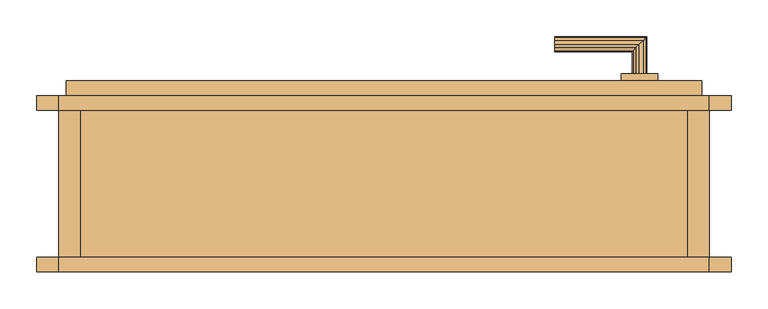
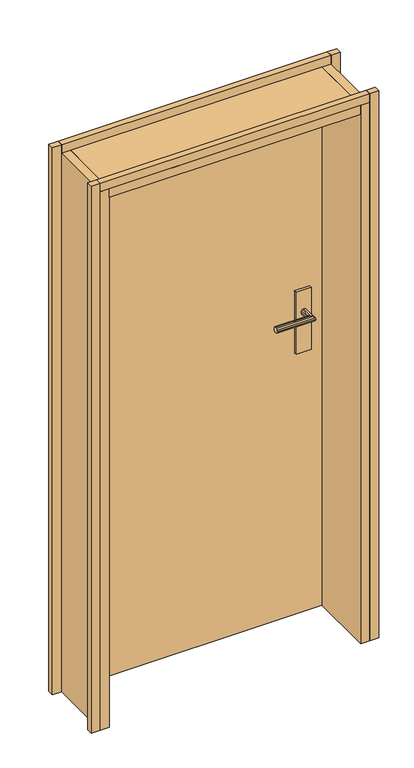
"""IFC4 building model written with IfcOpenShell, lengths in millimetres: door geometry, Tür."""

from ifc_helpers import new_model, si_unit, frame, origin, place, context, project, spatial, polyline, outline, extrude, faceted_brep, source, transform, mapped, element, save


def door_410d9d54(model_context):
    return source(origin(), model_context, "Body", "SolidModel", [
        extrude(outline(polyline([(855.0, 220.0), (855.0, -20.0), (30.0, -20.0), (30.0, 220.0), (855.0, 220.0)])), frame((0.0, 0.0, 1980.0), z_axis=(0.0, 0.0, 1.0), x_axis=(1.0, 0.0, 0.0)), (0.0, 0.0, 1.0), 30.0),
        extrude(outline(polyline([(765.0, 200.0), (815.0, 200.0), (815.0, 190.0), (765.0, 190.0), (765.0, 200.0)])), frame((0.0, 0.0, 1050.0), z_axis=(0.0, 0.0, 1.0), x_axis=(1.0, 0.0, 0.0)), (0.0, 0.0, 1.0), 215.0),
        extrude(outline(polyline([(915.0, 220.0), (915.0, 200.0), (885.0, 200.0), (885.0, 220.0), (915.0, 220.0)])), frame((0.0, 0.0, 140.0), z_axis=(0.0, 0.0, 1.0), x_axis=(1.0, 0.0, 0.0)), (0.0, 0.0, 1.0), 1900.0),
        extrude(outline(polyline([(30.0, 220.0), (30.0, -20.0), (0.0, -20.0), (0.0, 220.0), (30.0, 220.0)])), frame((0.0, 0.0, 140.0), z_axis=(0.0, 0.0, 1.0), x_axis=(1.0, 0.0, 0.0)), (0.0, 0.0, 1.0), 1870.0),
        extrude(outline(polyline([(915.0, 0.0), (915.0, -20.0), (885.0, -20.0), (885.0, 0.0), (915.0, 0.0)])), frame((0.0, 0.0, 140.0), z_axis=(0.0, 0.0, 1.0), x_axis=(1.0, 0.0, 0.0)), (0.0, 0.0, 1.0), 1900.0),
        extrude(outline(polyline([(815.0, 250.0), (815.0, 240.0), (765.0, 240.0), (765.0, 250.0), (815.0, 250.0)])), frame((0.0, 0.0, 1050.0), z_axis=(0.0, 0.0, 1.0), x_axis=(1.0, 0.0, 0.0)), (0.0, 0.0, 1.0), 215.0),
        faceted_brep([(795.0, 250.0, 1198.660254), (790.0, 250.0, 1200.0), (785.0, 250.0, 1198.660254), (781.339746, 250.0, 1195.0), (780.0, 250.0, 1190.0), (781.339746, 250.0, 1185.0), (785.0, 250.0, 1181.339746), (790.0, 250.0, 1180.0), (795.0, 250.0, 1181.339746), (798.660254, 250.0, 1185.0), (800.0, 250.0, 1190.0), (798.660254, 250.0, 1195.0), (790.0, 290.0, 1200.0), (795.0, 295.0, 1198.660254), (798.660254, 298.660254, 1195.0), (800.0, 300.0, 1190.0), (798.660254, 298.660254, 1185.0), (795.0, 295.0, 1181.339746), (790.0, 290.0, 1180.0), (785.0, 285.0, 1181.339746), (781.339746, 281.339746, 1185.0), (780.0, 280.0, 1190.0), (781.339746, 281.339746, 1195.0), (785.0, 285.0, 1198.660254), (675.0, 285.0, 1198.660254), (675.0, 290.0, 1200.0), (675.0, 295.0, 1198.660254), (675.0, 298.660254, 1195.0), (675.0, 300.0, 1190.0), (675.0, 298.660254, 1185.0), (675.0, 295.0, 1181.339746), (675.0, 290.0, 1180.0), (675.0, 285.0, 1181.339746), (675.0, 281.339746, 1185.0), (675.0, 280.0, 1190.0), (675.0, 281.339746, 1195.0)], [[[0, 1, 2, 3, 4, 5, 6, 7, 8, 9, 10, 11]], [[12, 1, 0, 13]], [[13, 0, 11, 14]], [[14, 11, 10, 15]], [[15, 10, 9, 16]], [[16, 9, 8, 17]], [[17, 8, 7, 18]], [[18, 7, 6, 19]], [[19, 6, 5, 20]], [[20, 5, 4, 21]], [[21, 4, 3, 22]], [[22, 3, 2, 23]], [[23, 2, 1, 12]], [[24, 25, 26, 27, 28, 29, 30, 31, 32, 33, 34, 35]], [[25, 12, 13, 26]], [[26, 13, 14, 27]], [[27, 14, 15, 28]], [[28, 15, 16, 29]], [[29, 16, 17, 30]], [[30, 17, 18, 31]], [[31, 18, 19, 32]], [[32, 19, 20, 33]], [[33, 20, 21, 34]], [[34, 21, 22, 35]], [[35, 22, 23, 24]], [[24, 23, 12, 25]]]),
        extrude(outline(polyline([(885.0, 220.0), (885.0, 200.0), (0.0, 200.0), (0.0, 220.0), (885.0, 220.0)])), frame((0.0, 0.0, 2010.0), z_axis=(0.0, 0.0, 1.0), x_axis=(1.0, 0.0, 0.0)), (0.0, 0.0, 1.0), 30.0),
        extrude(outline(polyline([(885.0, 0.0), (885.0, -20.0), (0.0, -20.0), (0.0, 0.0), (885.0, 0.0)])), frame((0.0, 0.0, 2010.0), z_axis=(0.0, 0.0, 1.0), x_axis=(1.0, 0.0, 0.0)), (0.0, 0.0, 1.0), 30.0),
        faceted_brep([(785.0, 190.0, 1198.660254), (790.0, 190.0, 1200.0), (795.0, 190.0, 1198.660254), (798.660254, 190.0, 1195.0), (800.0, 190.0, 1190.0), (798.660254, 190.0, 1185.0), (795.0, 190.0, 1181.339746), (790.0, 190.0, 1180.0), (785.0, 190.0, 1181.339746), (781.339746, 190.0, 1185.0), (780.0, 190.0, 1190.0), (781.339746, 190.0, 1195.0), (790.0, 150.0, 1200.0), (795.0, 145.0, 1198.660254), (798.660254, 141.339746, 1195.0), (800.0, 140.0, 1190.0), (798.660254, 141.339746, 1185.0), (795.0, 145.0, 1181.339746), (790.0, 150.0, 1180.0), (785.0, 155.0, 1181.339746), (781.339746, 158.660254, 1185.0), (780.0, 160.0, 1190.0), (781.339746, 158.660254, 1195.0), (785.0, 155.0, 1198.660254), (675.0, 145.0, 1198.660254), (675.0, 150.0, 1200.0), (675.0, 155.0, 1198.660254), (675.0, 158.660254, 1195.0), (675.0, 160.0, 1190.0), (675.0, 158.660254, 1185.0), (675.0, 155.0, 1181.339746), (675.0, 150.0, 1180.0), (675.0, 145.0, 1181.339746), (675.0, 141.339746, 1185.0), (675.0, 140.0, 1190.0), (675.0, 141.339746, 1195.0)], [[[0, 1, 2, 3, 4, 5, 6, 7, 8, 9, 10, 11]], [[2, 1, 12, 13]], [[3, 2, 13, 14]], [[4, 3, 14, 15]], [[5, 4, 15, 16]], [[6, 5, 16, 17]], [[7, 6, 17, 18]], [[8, 7, 18, 19]], [[9, 8, 19, 20]], [[10, 9, 20, 21]], [[11, 10, 21, 22]], [[0, 11, 22, 23]], [[1, 0, 23, 12]], [[24, 25, 26, 27, 28, 29, 30, 31, 32, 33, 34, 35]], [[13, 12, 25, 24]], [[14, 13, 24, 35]], [[15, 14, 35, 34]], [[16, 15, 34, 33]], [[17, 16, 33, 32]], [[18, 17, 32, 31]], [[19, 18, 31, 30]], [[20, 19, 30, 29]], [[21, 20, 29, 28]], [[22, 21, 28, 27]], [[23, 22, 27, 26]], [[12, 23, 26, 25]]]),
        extrude(outline(polyline([(875.0, 240.0), (875.0, 200.0), (10.0, 200.0), (10.0, 240.0), (875.0, 240.0)])), frame((0.0, 0.0, 140.0), z_axis=(0.0, 0.0, 1.0), x_axis=(1.0, 0.0, 0.0)), (0.0, 0.0, 1.0), 1860.0),
        extrude(outline(polyline([(885.0, 220.0), (885.0, -20.0), (855.0, -20.0), (855.0, 220.0), (885.0, 220.0)])), frame((0.0, 0.0, 140.0), z_axis=(0.0, 0.0, 1.0), x_axis=(1.0, 0.0, 0.0)), (0.0, 0.0, 1.0), 1870.0),
        extrude(outline(polyline([(0.0, -20.0), (-30.0, -20.0), (-30.0, 0.0), (0.0, 0.0), (0.0, -20.0)])), frame((0.0, 0.0, 140.0), z_axis=(0.0, 0.0, 1.0), x_axis=(1.0, 0.0, 0.0)), (0.0, 0.0, 1.0), 1900.0),
        extrude(outline(polyline([(0.0, 200.0), (-30.0, 200.0), (-30.0, 220.0), (0.0, 220.0), (0.0, 200.0)])), frame((0.0, 0.0, 140.0), z_axis=(0.0, 0.0, 1.0), x_axis=(1.0, 0.0, 0.0)), (0.0, 0.0, 1.0), 1900.0),
    ])


if __name__ == "__main__":
    model = new_model("IFC4")
    model_context = context("Model", 3, world=origin())
    ifc_project = project(units=[si_unit("LENGTHUNIT", "METRE", prefix="MILLI")], contexts=[model_context])
    site = spatial("IfcSite", under=ifc_project)
    building = spatial("IfcBuilding", under=site)
    placement = place(None, origin())
    door_shape = door_410d9d54(model_context)
    element("IfcDoor", 1, ObjectType="Tür", at=placement, inside=building, context=model_context, shape_type="MappedRepresentation", body=[
        mapped(door_shape, transform((0.0, 0.0, 0.0), x_axis=(1.0, 0.0, 0.0), y_axis=(0.0, 1.0, 0.0), z_axis=(0.0, 0.0, 1.0))),
    ])
    save(model, "model.ifc")

# Revit data of these elements
# Type "Tür"
#   Type Mark = "38"
# Element 1 (IfcDoor, "Tür")
#   Materials on its faces: "tuer_beschlag", "tuer_holzzarge"
# Materials
#   "tuer_beschlag": class "Unassigned", colour RGB 128 128 128, transparency 0
#   "tuer_holzzarge": class "Unassigned", colour RGB 255 255 255, transparency 0
